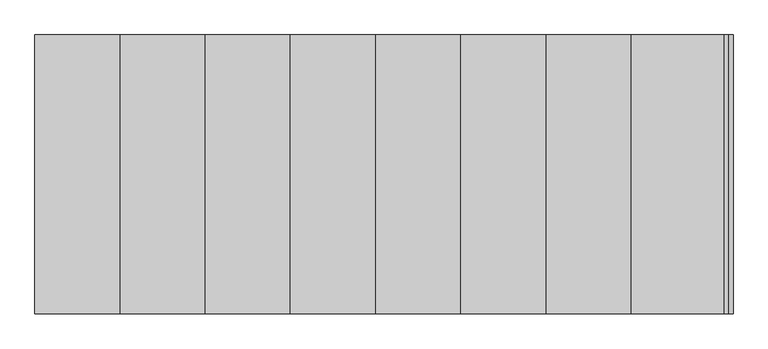
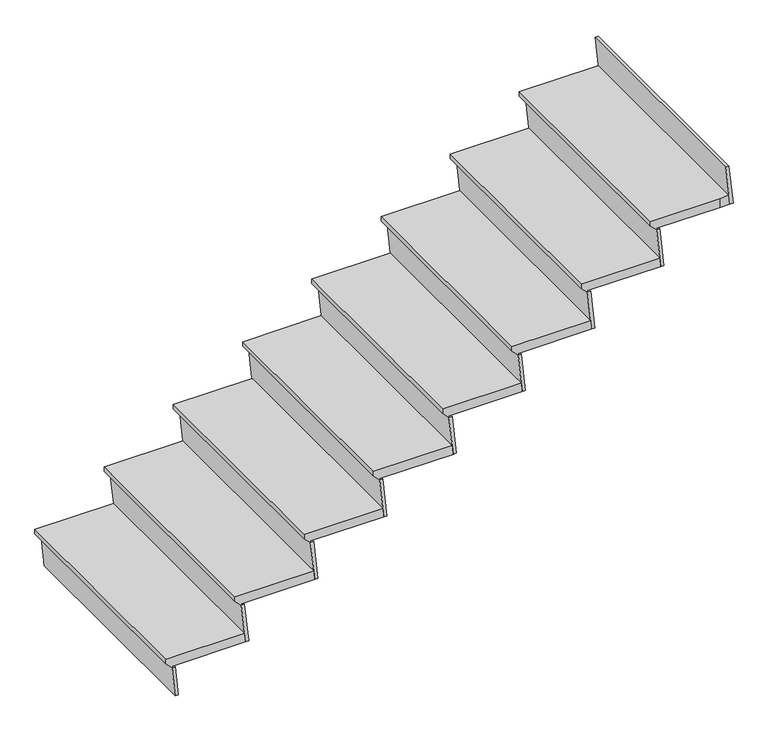
"""IFC4 building model written with IfcOpenShell, lengths in millimetres: stair flight geometry."""

import ifcopenshell
import ifcopenshell.guid

model = None  # the IFC model being written
_history = None  # IfcOwnerHistory: only IFC2X3 demands one
_inside = {}  # id of a spatial element -> (the spatial element, [elements in it])
_under = {}  # id of a project, library or spatial element -> (it, [spatial elements below it])
_declared = {}  # id of a project -> (the project, [libraries it declares])
_typed = {}  # id of a type object -> (the type object, [elements of that type])
_made_of = {}  # id of a material, layer set ... -> (it, [elements and type objects made of it])


def new_model(schema):
    """Start an empty IFC model of exactly this schema.

    Asked for "IFC4X3", IfcOpenShell would pick the latest addendum, in which some entities
    have other attributes; the version numbers below select the first issue.
    IFC2X3 requires an IfcOwnerHistory on every rooted entity: one is made here for all.
    """
    global model, _history
    if schema == "IFC4X3":
        model = ifcopenshell.file(schema_version=(4, 3, 0, 0))
    else:
        model = ifcopenshell.file(schema=schema)
    _inside.clear()
    _under.clear()
    _declared.clear()
    _typed.clear()
    _made_of.clear()
    _history = None
    if model.schema == "IFC2X3":
        org = make("IfcOrganization", Name="unknown")
        user = make(
            "IfcPersonAndOrganization",
            ThePerson=make("IfcPerson", FamilyName="unknown"),
            TheOrganization=org,
        )
        app = make(
            "IfcApplication",
            ApplicationDeveloper=org,
            Version="unknown",
            ApplicationFullName="unknown",
            ApplicationIdentifier="unknown",
        )
        _history = make(
            "IfcOwnerHistory",
            OwningUser=user,
            OwningApplication=app,
            ChangeAction="ADDED",
            CreationDate=0,
        )
    return model


def make(cls, **values):
    """One entity of the class cls with the attributes given. An attribute that is None is left unset."""
    return model.create_entity(
        cls, **{name: value for name, value in values.items() if value is not None}
    )


def rooted(cls, **values):
    """An entity with a GlobalId (a new one), such as an element, a storey or a relation."""
    return make(cls, GlobalId=ifcopenshell.guid.new(), OwnerHistory=_history, **values)


def si_unit(unit_type, name, prefix=None):
    """IfcSIUnit, for example si_unit("LENGTHUNIT", "METRE", prefix="MILLI")."""
    return make("IfcSIUnit", UnitType=unit_type, Prefix=prefix, Name=name)


def assignment(units):
    """IfcUnitAssignment: the units of a project."""
    return None if units is None else make("IfcUnitAssignment", Units=units)


def point(xyz):
    """IfcCartesianPoint."""
    return None if xyz is None else make("IfcCartesianPoint", Coordinates=xyz)


def direction(xyz):
    """IfcDirection."""
    return None if xyz is None else make("IfcDirection", DirectionRatios=xyz)


def frame(location, z_axis=None, x_axis=None):
    """IfcAxis2Placement3D, a coordinate frame: its origin and axes. An axis left out is left unset."""
    return make(
        "IfcAxis2Placement3D",
        Location=point(location),
        Axis=direction(z_axis),
        RefDirection=direction(x_axis),
    )


def origin():
    """The frame at (0, 0, 0) with its axes left unset."""
    return frame((0.0, 0.0, 0.0))


def place(relative_to, where):
    """IfcLocalPlacement: puts the frame where relative to a parent placement (None: the world)."""
    return make(
        "IfcLocalPlacement", PlacementRelTo=relative_to, RelativePlacement=where
    )


def context(
    kind, dimensions, precision=None, world=None, true_north=None, identifier=None
):
    """IfcGeometricRepresentationContext, for example the 3D "Model" context."""
    return make(
        "IfcGeometricRepresentationContext",
        ContextIdentifier=identifier,
        ContextType=kind,
        CoordinateSpaceDimension=dimensions,
        Precision=precision,
        WorldCoordinateSystem=world,
        TrueNorth=true_north,
    )


def project(units=None, contexts=None):
    """IfcProject with its units and contexts."""
    return rooted(
        "IfcProject",
        Name="project",
        RepresentationContexts=contexts,
        UnitsInContext=assignment(units),
    )


def spatial(cls, under=None, at=None, **own):
    """A site, building, storey or space (cls), placed at a placement, below another one or the project."""
    s = rooted(cls, ObjectPlacement=at, **own)
    if under is not None:
        _under.setdefault(under.id(), (under, []))[1].append(s)
    return s


def faces_of(points, faces, orient=None, outer=None):
    """IfcFace entities. A face is a list of loops; a loop is a list of indices into points, from 0.

    orient and outer hold one flag for each loop. By default every Orientation is true, the
    first loop of a face is its IfcFaceOuterBound and the others are IfcFaceBound.
    """
    made = []
    for i, loops in enumerate(faces):
        bounds = []
        for j, loop in enumerate(loops):
            is_outer = j == 0 if outer is None else outer[i][j]
            bounds.append(
                make(
                    "IfcFaceOuterBound" if is_outer else "IfcFaceBound",
                    Bound=make("IfcPolyLoop", Polygon=[points[k] for k in loop]),
                    Orientation=True if orient is None else orient[i][j],
                )
            )
        made.append(make("IfcFace", Bounds=bounds))
    return made


def faceted_brep(points, faces, orient=None, outer=None, voids=None):
    """IfcFacetedBrep: a solid bounded by flat faces; with voids (closed shells), ...WithVoids."""
    shared = [point(p) for p in points]
    hull = make("IfcClosedShell", CfsFaces=faces_of(shared, faces, orient, outer))
    if voids is None:
        return make("IfcFacetedBrep", Outer=hull)
    return make(
        "IfcFacetedBrepWithVoids",
        Outer=hull,
        Voids=[
            make(cls, CfsFaces=faces_of(shared, fs, o, b)) for cls, fs, o, b in voids
        ],
    )


def shape(context_of_items, identifier, shape_type, items):
    """IfcShapeRepresentation: the items that make up one representation, for example the "Body"."""
    return make(
        "IfcShapeRepresentation",
        ContextOfItems=context_of_items,
        RepresentationIdentifier=identifier,
        RepresentationType=shape_type,
        Items=items,
    )


def source(mapping_origin, context_of_items, identifier, shape_type, items):
    """IfcRepresentationMap: a shape defined once, which mapped items show again and again."""
    return make(
        "IfcRepresentationMap",
        MappingOrigin=mapping_origin,
        MappedRepresentation=shape(context_of_items, identifier, shape_type, items),
    )


def transform(
    local_origin,
    x_axis=None,
    y_axis=None,
    z_axis=None,
    scale=None,
    scale2=None,
    scale3=None,
    uniform=True,
):
    """IfcCartesianTransformationOperator3D, or its non-uniform kind. x_axis, y_axis, z_axis: its Axis1, 2, 3."""
    if uniform:
        return make(
            "IfcCartesianTransformationOperator3D",
            Axis1=direction(x_axis),
            Axis2=direction(y_axis),
            LocalOrigin=point(local_origin),
            Scale=scale,
            Axis3=direction(z_axis),
        )
    return make(
        "IfcCartesianTransformationOperator3DnonUniform",
        Axis1=direction(x_axis),
        Axis2=direction(y_axis),
        LocalOrigin=point(local_origin),
        Scale=scale,
        Axis3=direction(z_axis),
        Scale2=scale2,
        Scale3=scale3,
    )


def mapped(mapping_source, mapping_target):
    """IfcMappedItem: shows the shape of a source again, moved by a transform."""
    return make(
        "IfcMappedItem", MappingSource=mapping_source, MappingTarget=mapping_target
    )


def made_of(thing, what):
    """Note that an element or type object is made of a material, layer set ...; save() writes the relation."""
    if what is not None:
        _made_of.setdefault(what.id(), (what, []))[1].append(thing)
    return thing


def element(
    cls,
    number,
    at=None,
    inside=None,
    cuts=None,
    type_object=None,
    material=None,
    context=None,
    identifier="Body",
    shape_type=None,
    held_by="IfcProductDefinitionShape",
    body=None,
    shapes=None,
    **own,
):
    """One element of the class cls, such as IfcWall. Its Tag is "e" and its number.

    at: its placement. inside: the storey or other place that contains it. cuts: it is an
    opening in that element (IfcRelVoidsElement). A single representation is given by context,
    identifier, shape_type and body (its items); several are given by shapes. held_by: the class
    of the entity that holds the representations. save() writes the other relations.
    """
    e = rooted(cls, Tag="e%d" % number, ObjectPlacement=at, **own)
    if body is not None:
        shapes = [shape(context, identifier, shape_type, body)]
    if shapes is not None:
        e.Representation = make(held_by, Representations=shapes)
    if inside is not None:
        _inside.setdefault(inside.id(), (inside, []))[1].append(e)
    if cuts is not None:
        rooted(
            "IfcRelVoidsElement", RelatingBuildingElement=cuts, RelatedOpeningElement=e
        )
    if type_object is not None:
        _typed.setdefault(type_object.id(), (type_object, []))[1].append(e)
    return made_of(e, material)


def aggregate(whole, parts):
    """IfcRelAggregates: a whole, such as a stair, and the parts it consists of."""
    return rooted("IfcRelAggregates", RelatingObject=whole, RelatedObjects=parts)


def save(model, path):
    """Write the relations noted so far, then the file.

    IfcRelAggregates (storeys below a building ...), IfcRelContainedInSpatialStructure (elements
    in a storey), IfcRelDefinesByType, IfcRelAssociatesMaterial and IfcRelDeclares: one each for
    every whole, place, type object, material and project.
    """
    for whole, parts in _under.values():
        aggregate(whole, parts)
    for where, things in _inside.values():
        rooted(
            "IfcRelContainedInSpatialStructure",
            RelatedElements=things,
            RelatingStructure=where,
        )
    for kind, things in _typed.values():
        rooted("IfcRelDefinesByType", RelatedObjects=things, RelatingType=kind)
    for what, things in _made_of.values():
        rooted("IfcRelAssociatesMaterial", RelatedObjects=things, RelatingMaterial=what)
    for by, libraries in _declared.values():
        rooted("IfcRelDeclares", RelatingContext=by, RelatedDefinitions=libraries)
    model.write(path)


def stair_flight_35474383(model_context):
    return source(origin(), model_context, "Body", "Brep", [
        faceted_brep([(-17439.1481446, 16106.3635042, 169.3333333), (-17435.2735684, 16106.3635042, 131.2333333), (-17435.2735684, 17020.7635042, 131.2333333), (-17439.1481446, 17020.7635042, 169.3333333), (-17756.6481446, 17020.7635042, 169.3333333), (-17756.6481446, 16106.3635042, 169.3333333), (-17731.2481446, 16106.3635042, 131.2333333), (-17731.2481446, 17020.7635042, 131.2333333), (-17731.2481446, 17020.7635042, 124.8833333), (-17756.6481446, 17020.7635042, 150.2833333), (-17756.6481446, 16106.3635042, 150.2833333), (-17731.2481446, 16106.3635042, 124.8833333)], [[[0, 1, 2, 3]], [[4, 5, 0, 3]], [[2, 1, 6, 7]], [[4, 3, 2, 7, 8, 9]], [[0, 5, 10, 11, 6, 1]], [[10, 5, 4, 9]], [[11, 10, 9, 8]], [[11, 8, 7, 6]]]),
        faceted_brep([(-17731.2481446, 16106.3635042, 124.8833333), (-17718.5481446, 16106.3635042, 0.0), (-17705.7826428, 16106.3635042, 0.0), (-17718.4826428, 16106.3635042, 124.8833333), (-17731.2481446, 17020.7635042, 124.8833333), (-17718.4826428, 17020.7635042, 124.8833333), (-17705.7826428, 17020.7635042, 0.0), (-17718.5481446, 17020.7635042, 0.0)], [[[0, 1, 2, 3]], [[4, 5, 6, 7]], [[1, 0, 4, 7]], [[2, 1, 7, 6]], [[3, 2, 6, 5]], [[0, 3, 5, 4]]]),
        faceted_brep([(-17451.8481446, 16106.3635042, 294.2166667), (-17435.2735684, 16106.3635042, 131.2333333), (-17422.5080665, 16106.3635042, 131.2333333), (-17439.0826428, 16106.3635042, 294.2166667), (-17451.8481446, 17020.7635042, 294.2166667), (-17439.0826428, 17020.7635042, 294.2166667), (-17422.5080665, 17020.7635042, 131.2333333), (-17435.2735684, 17020.7635042, 131.2333333)], [[[0, 1, 2, 3]], [[4, 5, 6, 7]], [[1, 0, 4, 7]], [[2, 1, 7, 6]], [[3, 2, 6, 5]], [[0, 3, 5, 4]]]),
        faceted_brep([(-17477.2481446, 17020.7635042, 338.6666667), (-17477.2481446, 16106.3635042, 338.6666667), (-17159.7481446, 16106.3635042, 338.6666667), (-17159.7481446, 17020.7635042, 338.6666667), (-17155.8735684, 17020.7635042, 300.5666667), (-17155.8735684, 16106.3635042, 300.5666667), (-17451.8481446, 16106.3635042, 300.5666667), (-17451.8481446, 17020.7635042, 300.5666667), (-17451.8481446, 17020.7635042, 294.2166667), (-17477.2481446, 17020.7635042, 319.6166667), (-17477.2481446, 16106.3635042, 319.6166667), (-17451.8481446, 16106.3635042, 294.2166667)], [[[0, 1, 2, 3]], [[4, 5, 6, 7]], [[0, 3, 4, 7, 8, 9]], [[2, 1, 10, 11, 6, 5]], [[2, 5, 4, 3]], [[10, 1, 0, 9]], [[11, 10, 9, 8]], [[11, 8, 7, 6]]]),
        faceted_brep([(-17172.4481446, 16106.3635042, 463.55), (-17155.8735684, 16106.3635042, 300.5666667), (-17143.1080665, 16106.3635042, 300.5666667), (-17159.6826428, 16106.3635042, 463.55), (-17172.4481446, 17020.7635042, 463.55), (-17159.6826428, 17020.7635042, 463.55), (-17143.1080665, 17020.7635042, 300.5666667), (-17155.8735684, 17020.7635042, 300.5666667)], [[[0, 1, 2, 3]], [[4, 5, 6, 7]], [[1, 0, 4, 7]], [[2, 1, 7, 6]], [[3, 2, 6, 5]], [[0, 3, 5, 4]]]),
        faceted_brep([(-17197.8481446, 17020.7635042, 508.0), (-17197.8481446, 16106.3635042, 508.0), (-16880.3481446, 16106.3635042, 508.0), (-16880.3481446, 17020.7635042, 508.0), (-16876.4735684, 17020.7635042, 469.9), (-16876.4735684, 16106.3635042, 469.9), (-17172.4481446, 16106.3635042, 469.9), (-17172.4481446, 17020.7635042, 469.9), (-17172.4481446, 17020.7635042, 463.55), (-17197.8481446, 17020.7635042, 488.95), (-17197.8481446, 16106.3635042, 488.95), (-17172.4481446, 16106.3635042, 463.55)], [[[0, 1, 2, 3]], [[4, 5, 6, 7]], [[0, 3, 4, 7, 8, 9]], [[2, 1, 10, 11, 6, 5]], [[2, 5, 4, 3]], [[10, 1, 0, 9]], [[11, 10, 9, 8]], [[11, 8, 7, 6]]]),
        faceted_brep([(-16893.0481446, 16106.3635042, 632.8833333), (-16876.4735684, 16106.3635042, 469.9), (-16863.7080665, 16106.3635042, 469.9), (-16880.2826428, 16106.3635042, 632.8833333), (-16893.0481446, 17020.7635042, 632.8833333), (-16880.2826428, 17020.7635042, 632.8833333), (-16863.7080665, 17020.7635042, 469.9), (-16876.4735684, 17020.7635042, 469.9)], [[[0, 1, 2, 3]], [[4, 5, 6, 7]], [[1, 0, 4, 7]], [[2, 1, 7, 6]], [[3, 2, 6, 5]], [[0, 3, 5, 4]]]),
        faceted_brep([(-16918.4481446, 17020.7635042, 677.3333333), (-16918.4481446, 16106.3635042, 677.3333333), (-16600.9481446, 16106.3635042, 677.3333333), (-16600.9481446, 17020.7635042, 677.3333333), (-16597.0735684, 17020.7635042, 639.2333333), (-16597.0735684, 16106.3635042, 639.2333333), (-16893.0481446, 16106.3635042, 639.2333333), (-16893.0481446, 17020.7635042, 639.2333333), (-16893.0481446, 17020.7635042, 632.8833333), (-16918.4481446, 17020.7635042, 658.2833333), (-16918.4481446, 16106.3635042, 658.2833333), (-16893.0481446, 16106.3635042, 632.8833333)], [[[0, 1, 2, 3]], [[4, 5, 6, 7]], [[0, 3, 4, 7, 8, 9]], [[2, 1, 10, 11, 6, 5]], [[2, 5, 4, 3]], [[10, 1, 0, 9]], [[11, 10, 9, 8]], [[11, 8, 7, 6]]]),
        faceted_brep([(-16613.6481446, 16106.3635042, 802.2166667), (-16597.0735684, 16106.3635042, 639.2333333), (-16584.3080665, 16106.3635042, 639.2333333), (-16600.8826428, 16106.3635042, 802.2166667), (-16613.6481446, 17020.7635042, 802.2166667), (-16600.8826428, 17020.7635042, 802.2166667), (-16584.3080665, 17020.7635042, 639.2333333), (-16597.0735684, 17020.7635042, 639.2333333)], [[[0, 1, 2, 3]], [[4, 5, 6, 7]], [[1, 0, 4, 7]], [[2, 1, 7, 6]], [[3, 2, 6, 5]], [[0, 3, 5, 4]]]),
        faceted_brep([(-16639.0481446, 17020.7635042, 846.6666667), (-16639.0481446, 16106.3635042, 846.6666667), (-16321.5481446, 16106.3635042, 846.6666667), (-16321.5481446, 17020.7635042, 846.6666667), (-16317.6735684, 17020.7635042, 808.5666667), (-16317.6735684, 16106.3635042, 808.5666667), (-16613.6481446, 16106.3635042, 808.5666667), (-16613.6481446, 17020.7635042, 808.5666667), (-16613.6481446, 17020.7635042, 802.2166667), (-16639.0481446, 17020.7635042, 827.6166667), (-16639.0481446, 16106.3635042, 827.6166667), (-16613.6481446, 16106.3635042, 802.2166667)], [[[0, 1, 2, 3]], [[4, 5, 6, 7]], [[0, 3, 4, 7, 8, 9]], [[2, 1, 10, 11, 6, 5]], [[2, 5, 4, 3]], [[10, 1, 0, 9]], [[11, 10, 9, 8]], [[11, 8, 7, 6]]]),
        faceted_brep([(-16334.2481446, 16106.3635042, 971.55), (-16317.6735684, 16106.3635042, 808.5666667), (-16304.9080665, 16106.3635042, 808.5666667), (-16321.4826428, 16106.3635042, 971.55), (-16334.2481446, 17020.7635042, 971.55), (-16321.4826428, 17020.7635042, 971.55), (-16304.9080665, 17020.7635042, 808.5666667), (-16317.6735684, 17020.7635042, 808.5666667)], [[[0, 1, 2, 3]], [[4, 5, 6, 7]], [[1, 0, 4, 7]], [[2, 1, 7, 6]], [[3, 2, 6, 5]], [[0, 3, 5, 4]]]),
        faceted_brep([(-16359.6481446, 17020.7635042, 1016.0), (-16359.6481446, 16106.3635042, 1016.0), (-16042.1481446, 16106.3635042, 1016.0), (-16042.1481446, 17020.7635042, 1016.0), (-16038.2735684, 17020.7635042, 977.9), (-16038.2735684, 16106.3635042, 977.9), (-16334.2481446, 16106.3635042, 977.9), (-16334.2481446, 17020.7635042, 977.9), (-16334.2481446, 17020.7635042, 971.55), (-16359.6481446, 17020.7635042, 996.95), (-16359.6481446, 16106.3635042, 996.95), (-16334.2481446, 16106.3635042, 971.55)], [[[0, 1, 2, 3]], [[4, 5, 6, 7]], [[0, 3, 4, 7, 8, 9]], [[2, 1, 10, 11, 6, 5]], [[2, 5, 4, 3]], [[10, 1, 0, 9]], [[11, 10, 9, 8]], [[11, 8, 7, 6]]]),
        faceted_brep([(-16054.8481446, 16106.3635042, 1140.8833333), (-16038.2735684, 16106.3635042, 977.9), (-16025.5080665, 16106.3635042, 977.9), (-16042.0826428, 16106.3635042, 1140.8833333), (-16054.8481446, 17020.7635042, 1140.8833333), (-16042.0826428, 17020.7635042, 1140.8833333), (-16025.5080665, 17020.7635042, 977.9), (-16038.2735684, 17020.7635042, 977.9)], [[[0, 1, 2, 3]], [[4, 5, 6, 7]], [[1, 0, 4, 7]], [[2, 1, 7, 6]], [[3, 2, 6, 5]], [[0, 3, 5, 4]]]),
        faceted_brep([(-16080.2481446, 17020.7635042, 1185.3333333), (-16080.2481446, 16106.3635042, 1185.3333333), (-15762.7481446, 16106.3635042, 1185.3333333), (-15762.7481446, 17020.7635042, 1185.3333333), (-15758.8735684, 17020.7635042, 1147.2333333), (-15758.8735684, 16106.3635042, 1147.2333333), (-16054.8481446, 16106.3635042, 1147.2333333), (-16054.8481446, 17020.7635042, 1147.2333333), (-16054.8481446, 17020.7635042, 1140.8833333), (-16080.2481446, 17020.7635042, 1166.2833333), (-16080.2481446, 16106.3635042, 1166.2833333), (-16054.8481446, 16106.3635042, 1140.8833333)], [[[0, 1, 2, 3]], [[4, 5, 6, 7]], [[0, 3, 4, 7, 8, 9]], [[2, 1, 10, 11, 6, 5]], [[2, 5, 4, 3]], [[10, 1, 0, 9]], [[11, 10, 9, 8]], [[11, 8, 7, 6]]]),
        faceted_brep([(-15496.0481446, 16106.3635042, 1479.55), (-15479.4735684, 16106.3635042, 1316.5666667), (-15466.7080665, 16106.3635042, 1316.5666667), (-15483.2826428, 16106.3635042, 1479.55), (-15496.0481446, 17020.7635042, 1479.55), (-15483.2826428, 17020.7635042, 1479.55), (-15466.7080665, 17020.7635042, 1316.5666667), (-15479.4735684, 17020.7635042, 1316.5666667)], [[[0, 1, 2, 3]], [[4, 5, 6, 7]], [[1, 0, 4, 7]], [[2, 1, 7, 6]], [[3, 2, 6, 5]], [[0, 3, 5, 4]]]),
        faceted_brep([(-15775.4481446, 16106.3635042, 1310.2166667), (-15758.8735684, 16106.3635042, 1147.2333333), (-15746.1080665, 16106.3635042, 1147.2333333), (-15762.6826428, 16106.3635042, 1310.2166667), (-15775.4481446, 17020.7635042, 1310.2166667), (-15762.6826428, 17020.7635042, 1310.2166667), (-15746.1080665, 17020.7635042, 1147.2333333), (-15758.8735684, 17020.7635042, 1147.2333333)], [[[0, 1, 2, 3]], [[4, 5, 6, 7]], [[1, 0, 4, 7]], [[2, 1, 7, 6]], [[3, 2, 6, 5]], [[0, 3, 5, 4]]]),
        faceted_brep([(-15800.8481446, 17020.7635042, 1354.6666667), (-15800.8481446, 16106.3635042, 1354.6666667), (-15521.4481446, 16106.3635042, 1354.6666667), (-15483.3481446, 16106.3635042, 1354.6666667), (-15483.3481446, 17020.7635042, 1354.6666667), (-15521.4481446, 16106.3635042, 1316.5666667), (-15775.4481446, 16106.3635042, 1316.5666667), (-15775.4481446, 17020.7635042, 1316.5666667), (-15479.4735684, 17020.7635042, 1316.5666667), (-15479.4735684, 16106.3635042, 1316.5666667), (-15775.4481446, 17020.7635042, 1310.2166667), (-15800.8481446, 17020.7635042, 1335.6166667), (-15800.8481446, 16106.3635042, 1335.6166667), (-15775.4481446, 16106.3635042, 1310.2166667)], [[[0, 1, 2, 3, 4]], [[5, 6, 7, 8, 9]], [[0, 4, 8, 7, 10, 11]], [[2, 1, 12, 13, 6, 5]], [[3, 2, 5, 9]], [[3, 9, 8, 4]], [[12, 1, 0, 11]], [[13, 12, 11, 10]], [[13, 10, 7, 6]]]),
    ])


if __name__ == "__main__":
    model = new_model("IFC4")
    model_context = context("Model", 3, world=origin())
    ifc_project = project(units=[si_unit("LENGTHUNIT", "METRE", prefix="MILLI")], contexts=[model_context])
    site = spatial("IfcSite", under=ifc_project)
    building = spatial("IfcBuilding", under=site)
    placement = place(None, origin())
    stair_flight_shape = stair_flight_35474383(model_context)
    element("IfcStairFlight", 1, at=placement, inside=building, context=model_context, shape_type="MappedRepresentation", body=[
        mapped(stair_flight_shape, transform((0.0, 0.0, 0.0), x_axis=(1.0, 0.0, 0.0), y_axis=(0.0, 1.0, 0.0), z_axis=(0.0, 0.0, 1.0))),
    ])
    save(model, "model.ifc")

# Revit data of these elements
# Element 1 (IfcStairFlight)
#   Materials on its faces: "Concrete - Cast-in-Place Concrete", "Metal - Paint Finish - Dark Gray, Matte"
# Materials
#   "Concrete - Cast-in-Place Concrete": class "Unassigned", colour RGB 192 192 192, transparency 0
#   "Metal - Paint Finish - Dark Gray, Matte": class "Unassigned", colour RGB 98 98 98, transparency 0
